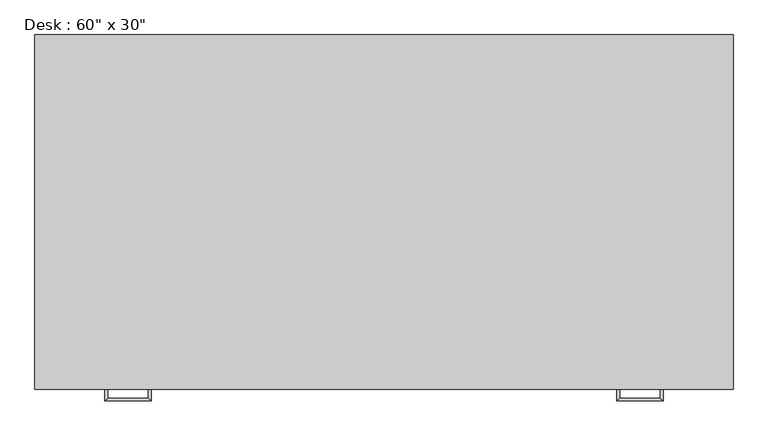
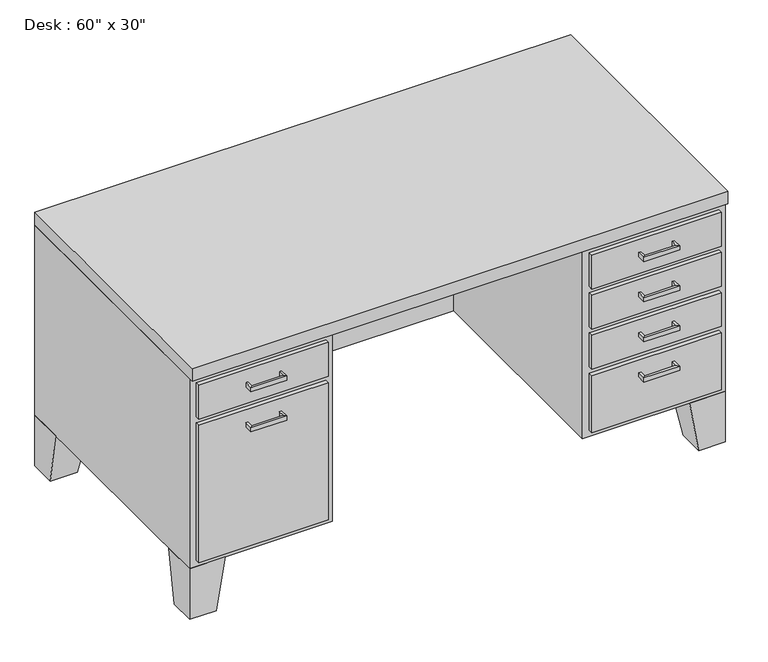
"""IFC4 building model written with IfcOpenShell, lengths in millimetres: furniture geometry."""

import ifcopenshell
import ifcopenshell.guid

model = None  # the IFC model being written
_history = None  # IfcOwnerHistory: only IFC2X3 demands one
_inside = {}  # id of a spatial element -> (the spatial element, [elements in it])
_under = {}  # id of a project, library or spatial element -> (it, [spatial elements below it])
_declared = {}  # id of a project -> (the project, [libraries it declares])
_typed = {}  # id of a type object -> (the type object, [elements of that type])
_made_of = {}  # id of a material, layer set ... -> (it, [elements and type objects made of it])


def new_model(schema):
    """Start an empty IFC model of exactly this schema.

    Asked for "IFC4X3", IfcOpenShell would pick the latest addendum, in which some entities
    have other attributes; the version numbers below select the first issue.
    IFC2X3 requires an IfcOwnerHistory on every rooted entity: one is made here for all.
    """
    global model, _history
    if schema == "IFC4X3":
        model = ifcopenshell.file(schema_version=(4, 3, 0, 0))
    else:
        model = ifcopenshell.file(schema=schema)
    _inside.clear()
    _under.clear()
    _declared.clear()
    _typed.clear()
    _made_of.clear()
    _history = None
    if model.schema == "IFC2X3":
        org = make("IfcOrganization", Name="unknown")
        user = make(
            "IfcPersonAndOrganization",
            ThePerson=make("IfcPerson", FamilyName="unknown"),
            TheOrganization=org,
        )
        app = make(
            "IfcApplication",
            ApplicationDeveloper=org,
            Version="unknown",
            ApplicationFullName="unknown",
            ApplicationIdentifier="unknown",
        )
        _history = make(
            "IfcOwnerHistory",
            OwningUser=user,
            OwningApplication=app,
            ChangeAction="ADDED",
            CreationDate=0,
        )
    return model


def make(cls, **values):
    """One entity of the class cls with the attributes given. An attribute that is None is left unset."""
    return model.create_entity(
        cls, **{name: value for name, value in values.items() if value is not None}
    )


def rooted(cls, **values):
    """An entity with a GlobalId (a new one), such as an element, a storey or a relation."""
    return make(cls, GlobalId=ifcopenshell.guid.new(), OwnerHistory=_history, **values)


def si_unit(unit_type, name, prefix=None):
    """IfcSIUnit, for example si_unit("LENGTHUNIT", "METRE", prefix="MILLI")."""
    return make("IfcSIUnit", UnitType=unit_type, Prefix=prefix, Name=name)


def assignment(units):
    """IfcUnitAssignment: the units of a project."""
    return None if units is None else make("IfcUnitAssignment", Units=units)


def point(xyz):
    """IfcCartesianPoint."""
    return None if xyz is None else make("IfcCartesianPoint", Coordinates=xyz)


def direction(xyz):
    """IfcDirection."""
    return None if xyz is None else make("IfcDirection", DirectionRatios=xyz)


def frame(location, z_axis=None, x_axis=None):
    """IfcAxis2Placement3D, a coordinate frame: its origin and axes. An axis left out is left unset."""
    return make(
        "IfcAxis2Placement3D",
        Location=point(location),
        Axis=direction(z_axis),
        RefDirection=direction(x_axis),
    )


def origin():
    """The frame at (0, 0, 0) with its axes left unset."""
    return frame((0.0, 0.0, 0.0))


def place(relative_to, where):
    """IfcLocalPlacement: puts the frame where relative to a parent placement (None: the world)."""
    return make(
        "IfcLocalPlacement", PlacementRelTo=relative_to, RelativePlacement=where
    )


def context(
    kind, dimensions, precision=None, world=None, true_north=None, identifier=None
):
    """IfcGeometricRepresentationContext, for example the 3D "Model" context."""
    return make(
        "IfcGeometricRepresentationContext",
        ContextIdentifier=identifier,
        ContextType=kind,
        CoordinateSpaceDimension=dimensions,
        Precision=precision,
        WorldCoordinateSystem=world,
        TrueNorth=true_north,
    )


def project(units=None, contexts=None):
    """IfcProject with its units and contexts."""
    return rooted(
        "IfcProject",
        Name="project",
        RepresentationContexts=contexts,
        UnitsInContext=assignment(units),
    )


def spatial(cls, under=None, at=None, **own):
    """A site, building, storey or space (cls), placed at a placement, below another one or the project."""
    s = rooted(cls, ObjectPlacement=at, **own)
    if under is not None:
        _under.setdefault(under.id(), (under, []))[1].append(s)
    return s


def polyline(points):
    """IfcPolyline through the points."""
    return make("IfcPolyline", Points=[point(p) for p in points])


def outline(outer, holes=None, kind="AREA"):
    """IfcArbitraryClosedProfileDef: a profile drawn as a closed curve; with holes, ...WithVoids."""
    if holes is None:
        return make("IfcArbitraryClosedProfileDef", ProfileType=kind, OuterCurve=outer)
    return make(
        "IfcArbitraryProfileDefWithVoids",
        ProfileType=kind,
        OuterCurve=outer,
        InnerCurves=holes,
    )


def extrude(swept, where, along, depth):
    """IfcExtrudedAreaSolid: the profile swept, set in the frame where, extruded along a direction by depth."""
    return make(
        "IfcExtrudedAreaSolid",
        SweptArea=swept,
        Position=where,
        ExtrudedDirection=direction(along),
        Depth=depth,
    )


def faces_of(points, faces, orient=None, outer=None):
    """IfcFace entities. A face is a list of loops; a loop is a list of indices into points, from 0.

    orient and outer hold one flag for each loop. By default every Orientation is true, the
    first loop of a face is its IfcFaceOuterBound and the others are IfcFaceBound.
    """
    made = []
    for i, loops in enumerate(faces):
        bounds = []
        for j, loop in enumerate(loops):
            is_outer = j == 0 if outer is None else outer[i][j]
            bounds.append(
                make(
                    "IfcFaceOuterBound" if is_outer else "IfcFaceBound",
                    Bound=make("IfcPolyLoop", Polygon=[points[k] for k in loop]),
                    Orientation=True if orient is None else orient[i][j],
                )
            )
        made.append(make("IfcFace", Bounds=bounds))
    return made


def faceted_brep(points, faces, orient=None, outer=None, voids=None):
    """IfcFacetedBrep: a solid bounded by flat faces; with voids (closed shells), ...WithVoids."""
    shared = [point(p) for p in points]
    hull = make("IfcClosedShell", CfsFaces=faces_of(shared, faces, orient, outer))
    if voids is None:
        return make("IfcFacetedBrep", Outer=hull)
    return make(
        "IfcFacetedBrepWithVoids",
        Outer=hull,
        Voids=[
            make(cls, CfsFaces=faces_of(shared, fs, o, b)) for cls, fs, o, b in voids
        ],
    )


def shape(context_of_items, identifier, shape_type, items):
    """IfcShapeRepresentation: the items that make up one representation, for example the "Body"."""
    return make(
        "IfcShapeRepresentation",
        ContextOfItems=context_of_items,
        RepresentationIdentifier=identifier,
        RepresentationType=shape_type,
        Items=items,
    )


def source(mapping_origin, context_of_items, identifier, shape_type, items):
    """IfcRepresentationMap: a shape defined once, which mapped items show again and again."""
    return make(
        "IfcRepresentationMap",
        MappingOrigin=mapping_origin,
        MappedRepresentation=shape(context_of_items, identifier, shape_type, items),
    )


def transform(
    local_origin,
    x_axis=None,
    y_axis=None,
    z_axis=None,
    scale=None,
    scale2=None,
    scale3=None,
    uniform=True,
):
    """IfcCartesianTransformationOperator3D, or its non-uniform kind. x_axis, y_axis, z_axis: its Axis1, 2, 3."""
    if uniform:
        return make(
            "IfcCartesianTransformationOperator3D",
            Axis1=direction(x_axis),
            Axis2=direction(y_axis),
            LocalOrigin=point(local_origin),
            Scale=scale,
            Axis3=direction(z_axis),
        )
    return make(
        "IfcCartesianTransformationOperator3DnonUniform",
        Axis1=direction(x_axis),
        Axis2=direction(y_axis),
        LocalOrigin=point(local_origin),
        Scale=scale,
        Axis3=direction(z_axis),
        Scale2=scale2,
        Scale3=scale3,
    )


def mapped(mapping_source, mapping_target):
    """IfcMappedItem: shows the shape of a source again, moved by a transform."""
    return make(
        "IfcMappedItem", MappingSource=mapping_source, MappingTarget=mapping_target
    )


def made_of(thing, what):
    """Note that an element or type object is made of a material, layer set ...; save() writes the relation."""
    if what is not None:
        _made_of.setdefault(what.id(), (what, []))[1].append(thing)
    return thing


def element(
    cls,
    number,
    at=None,
    inside=None,
    cuts=None,
    type_object=None,
    material=None,
    context=None,
    identifier="Body",
    shape_type=None,
    held_by="IfcProductDefinitionShape",
    body=None,
    shapes=None,
    **own,
):
    """One element of the class cls, such as IfcWall. Its Tag is "e" and its number.

    at: its placement. inside: the storey or other place that contains it. cuts: it is an
    opening in that element (IfcRelVoidsElement). A single representation is given by context,
    identifier, shape_type and body (its items); several are given by shapes. held_by: the class
    of the entity that holds the representations. save() writes the other relations.
    """
    e = rooted(cls, Tag="e%d" % number, ObjectPlacement=at, **own)
    if body is not None:
        shapes = [shape(context, identifier, shape_type, body)]
    if shapes is not None:
        e.Representation = make(held_by, Representations=shapes)
    if inside is not None:
        _inside.setdefault(inside.id(), (inside, []))[1].append(e)
    if cuts is not None:
        rooted(
            "IfcRelVoidsElement", RelatingBuildingElement=cuts, RelatedOpeningElement=e
        )
    if type_object is not None:
        _typed.setdefault(type_object.id(), (type_object, []))[1].append(e)
    return made_of(e, material)


def aggregate(whole, parts):
    """IfcRelAggregates: a whole, such as a stair, and the parts it consists of."""
    return rooted("IfcRelAggregates", RelatingObject=whole, RelatedObjects=parts)


def save(model, path):
    """Write the relations noted so far, then the file.

    IfcRelAggregates (storeys below a building ...), IfcRelContainedInSpatialStructure (elements
    in a storey), IfcRelDefinesByType, IfcRelAssociatesMaterial and IfcRelDeclares: one each for
    every whole, place, type object, material and project.
    """
    for whole, parts in _under.values():
        aggregate(whole, parts)
    for where, things in _inside.values():
        rooted(
            "IfcRelContainedInSpatialStructure",
            RelatedElements=things,
            RelatingStructure=where,
        )
    for kind, things in _typed.values():
        rooted("IfcRelDefinesByType", RelatedObjects=things, RelatingType=kind)
    for what, things in _made_of.values():
        rooted("IfcRelAssociatesMaterial", RelatedObjects=things, RelatingMaterial=what)
    for by, libraries in _declared.values():
        rooted("IfcRelDeclares", RelatingContext=by, RelatedDefinitions=libraries)
    model.write(path)


def furniture_f1eb905c(model_context):
    return source(origin(), model_context, "Body", "SolidModel", [
        extrude(outline(polyline([(19.05, 0.0), (387.35, 0.0), (387.35, -12.7), (19.05, -12.7), (19.05, 0.0)])), frame((0.0, 0.0, 603.25), z_axis=(0.0, 0.0, 1.0), x_axis=(1.0, 0.0, 0.0)), (0.0, 0.0, 1.0), 101.6),
        extrude(outline(polyline([(19.05, 0.0), (387.35, 0.0), (387.35, -12.7), (19.05, -12.7), (19.05, 0.0)])), frame((0.0, 0.0, 171.45), z_axis=(0.0, 0.0, 1.0), x_axis=(1.0, 0.0, 0.0)), (0.0, 0.0, 1.0), 412.75),
        extrude(outline(polyline([(1136.65, 0.0), (1504.95, 0.0), (1504.95, -12.7), (1136.65, -12.7), (1136.65, 0.0)])), frame((0.0, 0.0, 603.25), z_axis=(0.0, 0.0, 1.0), x_axis=(1.0, 0.0, 0.0)), (0.0, 0.0, 1.0), 101.6),
        extrude(outline(polyline([(1136.65, 0.0), (1504.95, 0.0), (1504.95, -12.7), (1136.65, -12.7), (1136.65, 0.0)])), frame((0.0, 0.0, 171.45), z_axis=(0.0, 0.0, 1.0), x_axis=(1.0, 0.0, 0.0)), (0.0, 0.0, 1.0), 171.45),
        extrude(outline(polyline([(1136.65, 0.0), (1504.95, 0.0), (1504.95, -12.7), (1136.65, -12.7), (1136.65, 0.0)])), frame((0.0, 0.0, 482.6), z_axis=(0.0, 0.0, 1.0), x_axis=(1.0, 0.0, 0.0)), (0.0, 0.0, 1.0), 101.6),
        extrude(outline(polyline([(1136.65, 0.0), (1504.95, 0.0), (1504.95, -12.7), (1136.65, -12.7), (1136.65, 0.0)])), frame((0.0, 0.0, 361.95), z_axis=(0.0, 0.0, 1.0), x_axis=(1.0, 0.0, 0.0)), (0.0, 0.0, 1.0), 101.6),
        faceted_brep([(101.6, 0.0, 152.4), (101.6, 101.6, 152.4), (0.0, 101.6, 152.4), (0.0, 0.0, 152.4), (76.2, 0.0, 0.0), (0.0, 0.0, 0.0), (0.0, 76.2, 0.0), (76.2, 76.2, 0.0)], [[[0, 1, 2, 3]], [[4, 5, 6, 7]], [[4, 7, 1, 0]], [[7, 6, 2, 1]], [[6, 5, 3, 2]], [[5, 4, 0, 3]]]),
        faceted_brep([(101.6, 762.0, 152.4), (0.0, 762.0, 152.4), (0.0, 660.4, 152.4), (101.6, 660.4, 152.4), (76.2, 762.0, 0.0), (76.2, 685.8, 0.0), (0.0, 685.8, 0.0), (0.0, 762.0, 0.0)], [[[0, 1, 2, 3]], [[4, 5, 6, 7]], [[4, 7, 1, 0]], [[7, 6, 2, 1]], [[6, 5, 3, 2]], [[5, 4, 0, 3]]]),
        faceted_brep([(1422.4, 762.0, 152.4), (1422.4, 660.4, 152.4), (1524.0, 660.4, 152.4), (1524.0, 762.0, 152.4), (1447.8, 762.0, 0.0), (1524.0, 762.0, 0.0), (1524.0, 685.8, 0.0), (1447.8, 685.8, 0.0)], [[[0, 1, 2, 3]], [[4, 5, 6, 7]], [[4, 7, 1, 0]], [[7, 6, 2, 1]], [[6, 5, 3, 2]], [[5, 4, 0, 3]]]),
        faceted_brep([(1422.4, 0.0, 152.4), (1524.0, 0.0, 152.4), (1524.0, 101.6, 152.4), (1422.4, 101.6, 152.4), (1447.8, 0.0, 0.0), (1447.8, 76.2, 0.0), (1524.0, 76.2, 0.0), (1524.0, 0.0, 0.0)], [[[0, 1, 2, 3]], [[4, 5, 6, 7]], [[4, 7, 1, 0]], [[7, 6, 2, 1]], [[6, 5, 3, 2]], [[5, 4, 0, 3]]]),
        extrude(outline(polyline([(0.0, -12.7), (0.0, 762.0), (1524.0, 762.0), (1524.0, -12.7), (0.0, -12.7)])), frame((0.0, 0.0, 723.9), z_axis=(0.0, 0.0, 1.0), x_axis=(1.0, 0.0, 0.0)), (0.0, 0.0, 1.0), 38.1),
        extrude(outline(polyline([(1117.6, 0.0), (1117.6, 635.0), (406.4, 635.0), (406.4, 0.0), (0.0, 0.0), (0.0, 762.0), (1524.0, 762.0), (1524.0, 0.0), (1117.6, 0.0)])), frame((0.0, 0.0, 152.4), z_axis=(0.0, 0.0, 1.0), x_axis=(1.0, 0.0, 0.0)), (0.0, 0.0, 1.0), 571.5),
        faceted_brep([(158.75, -12.7, 546.1), (158.75, -12.7, 533.4), (152.4, -12.7, 533.4), (152.4, -12.7, 546.1), (158.75, -31.75, 546.1), (158.75, -31.75, 533.4), (152.4, -38.1, 533.4), (152.4, -38.1, 546.1), (247.65, -31.75, 546.1), (247.65, -31.75, 533.4), (254.0, -38.1, 533.4), (254.0, -38.1, 546.1), (247.65, -12.7, 546.1), (254.0, -12.7, 546.1), (254.0, -12.7, 533.4), (247.65, -12.7, 533.4)], [[[0, 1, 2, 3]], [[1, 0, 4, 5]], [[2, 1, 5, 6]], [[3, 2, 6, 7]], [[0, 3, 7, 4]], [[5, 4, 8, 9]], [[6, 5, 9, 10]], [[7, 6, 10, 11]], [[4, 7, 11, 8]], [[12, 13, 14, 15]], [[9, 8, 12, 15]], [[10, 9, 15, 14]], [[11, 10, 14, 13]], [[8, 11, 13, 12]]]),
        faceted_brep([(158.75, -12.7, 666.75), (158.75, -12.7, 654.05), (152.4, -12.7, 654.05), (152.4, -12.7, 666.75), (158.75, -31.75, 666.75), (158.75, -31.75, 654.05), (152.4, -38.1, 654.05), (152.4, -38.1, 666.75), (247.65, -31.75, 666.75), (247.65, -31.75, 654.05), (254.0, -38.1, 654.05), (254.0, -38.1, 666.75), (247.65, -12.7, 666.75), (254.0, -12.7, 666.75), (254.0, -12.7, 654.05), (247.65, -12.7, 654.05)], [[[0, 1, 2, 3]], [[1, 0, 4, 5]], [[2, 1, 5, 6]], [[3, 2, 6, 7]], [[0, 3, 7, 4]], [[5, 4, 8, 9]], [[6, 5, 9, 10]], [[7, 6, 10, 11]], [[4, 7, 11, 8]], [[12, 13, 14, 15]], [[9, 8, 12, 15]], [[10, 9, 15, 14]], [[11, 10, 14, 13]], [[8, 11, 13, 12]]]),
        faceted_brep([(1365.25, -12.7, 304.8), (1371.6, -12.7, 304.8), (1371.6, -12.7, 292.1), (1365.25, -12.7, 292.1), (1365.25, -31.75, 304.8), (1371.6, -38.1, 304.8), (1371.6, -38.1, 292.1), (1365.25, -31.75, 292.1), (1276.35, -31.75, 304.8), (1270.0, -38.1, 304.8), (1270.0, -38.1, 292.1), (1276.35, -31.75, 292.1), (1276.35, -12.7, 304.8), (1276.35, -12.7, 292.1), (1270.0, -12.7, 292.1), (1270.0, -12.7, 304.8)], [[[0, 1, 2, 3]], [[1, 0, 4, 5]], [[2, 1, 5, 6]], [[3, 2, 6, 7]], [[0, 3, 7, 4]], [[5, 4, 8, 9]], [[6, 5, 9, 10]], [[7, 6, 10, 11]], [[4, 7, 11, 8]], [[12, 13, 14, 15]], [[9, 8, 12, 15]], [[10, 9, 15, 14]], [[11, 10, 14, 13]], [[8, 11, 13, 12]]]),
        faceted_brep([(1365.25, -12.7, 425.45), (1371.6, -12.7, 425.45), (1371.6, -12.7, 412.75), (1365.25, -12.7, 412.75), (1365.25, -31.75, 425.45), (1371.6, -38.1, 425.45), (1371.6, -38.1, 412.75), (1365.25, -31.75, 412.75), (1276.35, -31.75, 425.45), (1270.0, -38.1, 425.45), (1270.0, -38.1, 412.75), (1276.35, -31.75, 412.75), (1276.35, -12.7, 425.45), (1276.35, -12.7, 412.75), (1270.0, -12.7, 412.75), (1270.0, -12.7, 425.45)], [[[0, 1, 2, 3]], [[1, 0, 4, 5]], [[2, 1, 5, 6]], [[3, 2, 6, 7]], [[0, 3, 7, 4]], [[5, 4, 8, 9]], [[6, 5, 9, 10]], [[7, 6, 10, 11]], [[4, 7, 11, 8]], [[12, 13, 14, 15]], [[9, 8, 12, 15]], [[10, 9, 15, 14]], [[11, 10, 14, 13]], [[8, 11, 13, 12]]]),
        faceted_brep([(1365.25, -12.7, 546.1), (1371.6, -12.7, 546.1), (1371.6, -12.7, 533.4), (1365.25, -12.7, 533.4), (1365.25, -31.75, 546.1), (1371.6, -38.1, 546.1), (1371.6, -38.1, 533.4), (1365.25, -31.75, 533.4), (1276.35, -31.75, 546.1), (1270.0, -38.1, 546.1), (1270.0, -38.1, 533.4), (1276.35, -31.75, 533.4), (1276.35, -12.7, 546.1), (1276.35, -12.7, 533.4), (1270.0, -12.7, 533.4), (1270.0, -12.7, 546.1)], [[[0, 1, 2, 3]], [[1, 0, 4, 5]], [[2, 1, 5, 6]], [[3, 2, 6, 7]], [[0, 3, 7, 4]], [[5, 4, 8, 9]], [[6, 5, 9, 10]], [[7, 6, 10, 11]], [[4, 7, 11, 8]], [[12, 13, 14, 15]], [[9, 8, 12, 15]], [[10, 9, 15, 14]], [[11, 10, 14, 13]], [[8, 11, 13, 12]]]),
        faceted_brep([(1365.25, -12.7, 666.75), (1371.6, -12.7, 666.75), (1371.6, -12.7, 654.05), (1365.25, -12.7, 654.05), (1365.25, -31.75, 666.75), (1371.6, -38.1, 666.75), (1371.6, -38.1, 654.05), (1365.25, -31.75, 654.05), (1276.35, -31.75, 666.75), (1270.0, -38.1, 666.75), (1270.0, -38.1, 654.05), (1276.35, -31.75, 654.05), (1276.35, -12.7, 666.75), (1276.35, -12.7, 654.05), (1270.0, -12.7, 654.05), (1270.0, -12.7, 666.75)], [[[0, 1, 2, 3]], [[1, 0, 4, 5]], [[2, 1, 5, 6]], [[3, 2, 6, 7]], [[0, 3, 7, 4]], [[5, 4, 8, 9]], [[6, 5, 9, 10]], [[7, 6, 10, 11]], [[4, 7, 11, 8]], [[12, 13, 14, 15]], [[9, 8, 12, 15]], [[10, 9, 15, 14]], [[11, 10, 14, 13]], [[8, 11, 13, 12]]]),
    ])


if __name__ == "__main__":
    model = new_model("IFC4")
    model_context = context("Model", 3, world=origin())
    ifc_project = project(units=[si_unit("LENGTHUNIT", "METRE", prefix="MILLI")], contexts=[model_context])
    site = spatial("IfcSite", under=ifc_project)
    building = spatial("IfcBuilding", under=site)
    placement = place(None, origin())
    furniture_shape = furniture_f1eb905c(model_context)
    element("IfcFurniture", 1, ObjectType="Desk : 60\" x 30\"", at=placement, inside=building, context=model_context, shape_type="MappedRepresentation", body=[
        mapped(furniture_shape, transform((0.0, 0.0, 0.0), x_axis=(1.0, 0.0, 0.0), y_axis=(0.0, 1.0, 0.0), z_axis=(0.0, 0.0, 1.0))),
    ])
    save(model, "model.ifc")

# Revit data of these elements
# Type "Desk : 60\" x 30\""
#   Assembly Code = "E2020200"
#   Depth = 2' - 6"
#   Height = 2' - 6"
#   Leg Height = 0' - 6"
#   Width = 5' - 0"
#   Body Material = Laminate, Ivory, Matte
#   Handle/Leg Material = Steel, Chrome Plated
#   Top Material = Cherry
#   Default Elevation = 0
# Element 1 (IfcFurniture, "Desk : 60\" x 30\"")
#   Materials on its faces: "Steel, Chrome Plated", "Laminate, Ivory, Matte", "Cherry"
# Materials
#   "Laminate, Ivory, Matte": class "Plastic", colour RGB 247 247 239, transparency 0, Description = "Plastic Laminate - Ivory, Matte", Cost = 0
#   "Steel, Chrome Plated": class "Metal", colour RGB 17 17 17, transparency 0, Description = "Chromiuim plated steel", Cost = 0
#   "Cherry": class "Wood", colour RGB 226 177 128, transparency 0, Description = "Prunus Serotina", Cost = 0
